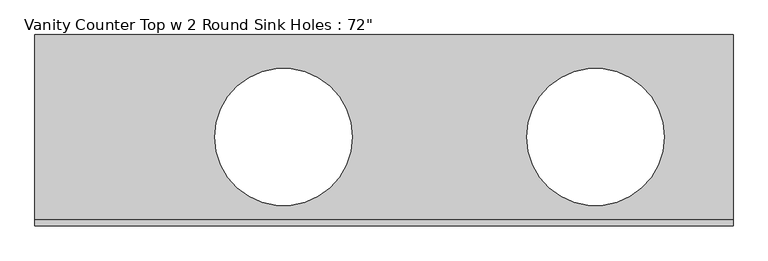
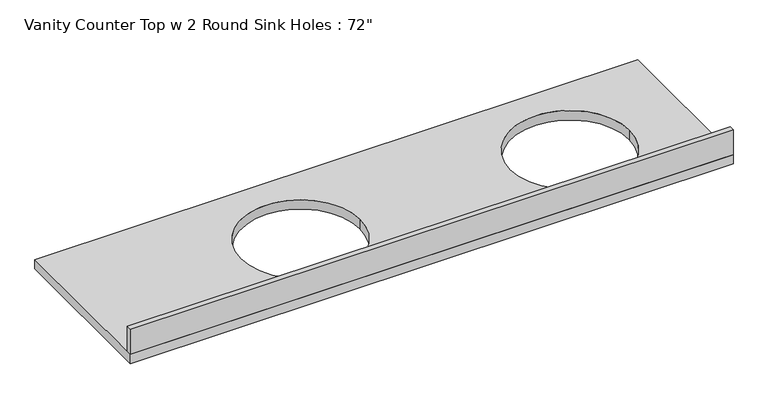
"""IFC4 building model written with IfcOpenShell, lengths in millimetres: furniture geometry."""

from ifc_helpers import new_model, si_unit, point, frame, frame_2d, origin, place, context, project, spatial, polyline, circle_curve, trimmed, segment, composite_curve, outline, extrude, source, transform, mapped, element, save


def furniture_36b949cc(model_context):
    return source(origin(), model_context, "Body", "SweptSolid", [
        extrude(outline(polyline([(-1327.4622951, 0.0), (-1327.4622951, 19.05), (991.4783299, 19.05), (991.4783299, 0.0), (-1327.4622951, 0.0)])), frame((0.0, 0.0, 787.4), z_axis=(0.0, 0.0, 1.0), x_axis=(1.0, 0.0, 0.0)), (0.0, 0.0, 1.0), 101.6),
        extrude(outline(polyline([(991.4783299, 0.0), (-1327.4622951, 0.0), (-1327.4622951, 635.0), (991.4783299, 635.0), (991.4783299, 0.0)]), holes=[composite_curve([segment(trimmed(circle_curve(frame_2d((-501.9622951, 295.275)), 228.6), [point((-730.5622951, 295.275))], [point((-273.3622951, 295.275))], True, "CARTESIAN"), True, "CONTINUOUS"), segment(trimmed(circle_curve(frame_2d((-501.9622951, 295.275)), 228.6), [point((-273.3622951, 295.275))], [point((-730.5622951, 295.275))], True, "CARTESIAN"), True, "CONTINUOUS")], self_intersect=False), composite_curve([segment(trimmed(circle_curve(frame_2d((534.2783299, 295.275)), 228.6), [point((305.6783299, 295.275))], [point((762.8783299, 295.275))], True, "CARTESIAN"), True, "CONTINUOUS"), segment(trimmed(circle_curve(frame_2d((534.2783299, 295.275)), 228.6), [point((762.8783299, 295.275))], [point((305.6783299, 295.275))], True, "CARTESIAN"), True, "CONTINUOUS")], self_intersect=False)]), frame((0.0, 0.0, 749.3), z_axis=(0.0, 0.0, 1.0), x_axis=(1.0, 0.0, 0.0)), (0.0, 0.0, 1.0), 38.1),
    ])


if __name__ == "__main__":
    model = new_model("IFC4")
    model_context = context("Model", 3, world=origin())
    ifc_project = project(units=[si_unit("LENGTHUNIT", "METRE", prefix="MILLI")], contexts=[model_context])
    site = spatial("IfcSite", under=ifc_project)
    building = spatial("IfcBuilding", under=site)
    placement = place(None, origin())
    furniture_shape = furniture_36b949cc(model_context)
    element("IfcFurniture", 1, ObjectType="Vanity Counter Top w 2 Round Sink Holes : 72\"", at=placement, inside=building, context=model_context, shape_type="MappedRepresentation", body=[
        mapped(furniture_shape, transform((0.0, 0.0, 0.0), x_axis=(1.0, 0.0, 0.0), y_axis=(0.0, 1.0, 0.0), z_axis=(0.0, 0.0, 1.0))),
    ])
    save(model, "model.ifc")

# Revit data of these elements
# Type "Vanity Counter Top w 2 Round Sink Holes : 72\""
#   Assembly Code = "C1030400"
#   Sink Location Right = 1' - 6"
#   Counter Thickness = 0' - 1 1/2"
#   Depth = 2' - 1"
#   Height = 2' - 7"
#   Length [instance default] = 6' - 0"
#   Sink Location Left [instance default] = 1' - 6"
#   Sink Location To Wall [instance default] = 0' - 4"
#   Sink Opening Width [instance default] = 1' - 5"
#   Counter Top = Counter Top
# Element 1 (IfcFurniture, "Vanity Counter Top w 2 Round Sink Holes : 72\"")
#   Length = 7' - 7 19/64"
#   Sink Location Left = 2' - 8 1/2"
#   Sink Location To Wall = 0' - 3 1/8"
#   Materials on its faces: "Counter Top"
# Materials
#   "Counter Top": class "Wood", colour RGB 226 177 128, transparency 0
